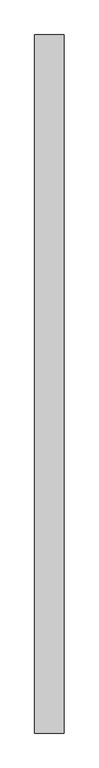
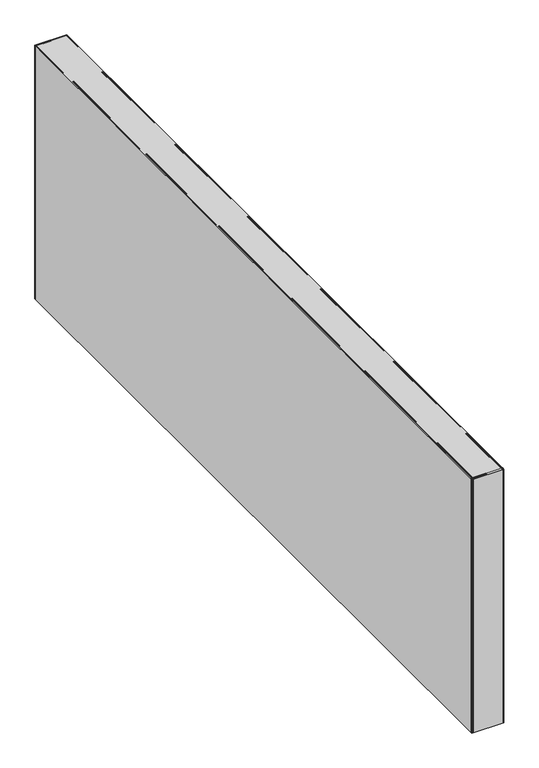
"""IFC4 building model written with IfcOpenShell, lengths in millimetres: beam geometry, LF02ZBK001_DIKE WALL_RC : Dike_Thk.250_EW3."""

from ifc_helpers import new_model, si_unit, origin, origin_with_axes, place, context, project, spatial, polyline, outline, extrude, source, transform, mapped, element, save


def beam_991fab6d(model_context):
    return source(origin(), model_context, "Body", "SweptSolid", [
        extrude(outline(polyline([(125.0, -2965.0), (-125.0, -2965.0), (-125.0, 2965.0), (125.0, 2965.0), (125.0, -2965.0)])), origin_with_axes(), (0.0, 0.0, 1.0), 2100.0),
        extrude(outline(polyline([(-125.0, -2950.0), (-125.0, -2949.0), (125.0, -2949.0), (125.0, -2950.0), (-125.0, -2950.0)])), origin_with_axes(), (0.0, 0.0, 1.0), 2100.0),
        extrude(outline(polyline([(-125.0, -2955.0), (-125.0, -2954.0), (125.0, -2954.0), (125.0, -2955.0), (-125.0, -2955.0)])), origin_with_axes(), (0.0, 0.0, 1.0), 2100.0),
        extrude(outline(polyline([(-125.0, -2960.0), (-125.0, -2959.0), (125.0, -2959.0), (125.0, -2960.0), (-125.0, -2960.0)])), origin_with_axes(), (0.0, 0.0, 1.0), 2100.0),
        extrude(outline(polyline([(-125.0, 2950.0), (125.0, 2950.0), (125.0, 2949.0), (-125.0, 2949.0), (-125.0, 2950.0)])), origin_with_axes(), (0.0, 0.0, 1.0), 2100.0),
        extrude(outline(polyline([(-125.0, 2955.0), (125.0, 2955.0), (125.0, 2954.0), (-125.0, 2954.0), (-125.0, 2955.0)])), origin_with_axes(), (0.0, 0.0, 1.0), 2100.0),
        extrude(outline(polyline([(-125.0, 2960.0), (125.0, 2960.0), (125.0, 2959.0), (-125.0, 2959.0), (-125.0, 2960.0)])), origin_with_axes(), (0.0, 0.0, 1.0), 2100.0),
        extrude(outline(polyline([(109.0, 2965.0), (110.0, 2965.0), (110.0, -2965.0), (109.0, -2965.0), (109.0, 2965.0)])), origin_with_axes(), (0.0, 0.0, 1.0), 2100.0),
        extrude(outline(polyline([(114.0, 2965.0), (115.0, 2965.0), (115.0, -2965.0), (114.0, -2965.0), (114.0, 2965.0)])), origin_with_axes(), (0.0, 0.0, 1.0), 2100.0),
        extrude(outline(polyline([(119.0, 2965.0), (120.0, 2965.0), (120.0, -2965.0), (119.0, -2965.0), (119.0, 2965.0)])), origin_with_axes(), (0.0, 0.0, 1.0), 2100.0),
        extrude(outline(polyline([(-109.0, 2965.0), (-109.0, -2965.0), (-110.0, -2965.0), (-110.0, 2965.0), (-109.0, 2965.0)])), origin_with_axes(), (0.0, 0.0, 1.0), 2100.0),
        extrude(outline(polyline([(-114.0, 2965.0), (-114.0, -2965.0), (-115.0, -2965.0), (-115.0, 2965.0), (-114.0, 2965.0)])), origin_with_axes(), (0.0, 0.0, 1.0), 2100.0),
        extrude(outline(polyline([(-119.0, 2965.0), (-119.0, -2965.0), (-120.0, -2965.0), (-120.0, 2965.0), (-119.0, 2965.0)])), origin_with_axes(), (0.0, 0.0, 1.0), 2100.0),
    ])


if __name__ == "__main__":
    model = new_model("IFC4")
    model_context = context("Model", 3, world=origin())
    ifc_project = project(units=[si_unit("LENGTHUNIT", "METRE", prefix="MILLI")], contexts=[model_context])
    site = spatial("IfcSite", under=ifc_project)
    building = spatial("IfcBuilding", under=site)
    placement = place(None, origin())
    beam_shape = beam_991fab6d(model_context)
    element("IfcBeam", 1, ObjectType="LF02ZBK001_DIKE WALL_RC : Dike_Thk.250_EW3", at=placement, inside=building, context=model_context, shape_type="MappedRepresentation", body=[
        mapped(beam_shape, transform((0.0, 0.0, 0.0), x_axis=(1.0, 0.0, 0.0), y_axis=(0.0, 1.0, 0.0), z_axis=(0.0, 0.0, 1.0))),
    ])
    save(model, "model.ifc")

# Revit data of these elements
# Type "LF02ZBK001_DIKE WALL_RC : Dike_Thk.250_EW3"
#   Dike_thk = 250 mm
#   Dike_Length [instance default] = 3000 mm
#   Dike_Hight = 2100 mm
#   c2_visible = yes
#   c3_material [instance default] = none
#   c2_material 3 [instance default] = none
#   c2_material 2 [instance default] = none
#   c2_material 1 [instance default] = none
#   c1_material [instance default] = none
#   Default Elevation = 0
# Element 1 (IfcBeam, "LF02ZBK001_DIKE WALL_RC : Dike_Thk.250_EW3")
#   Dike_Length = 5930 mm
